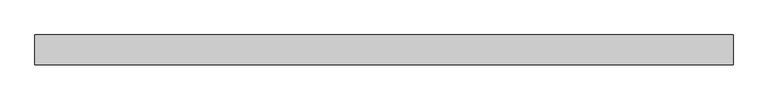
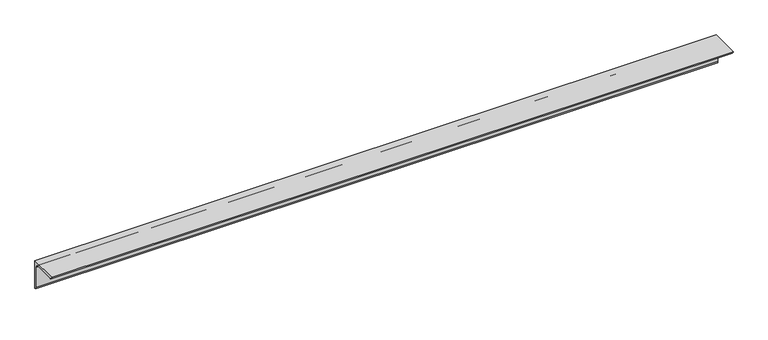
"""IFC4 building model written with IfcOpenShell, lengths in millimetres: beam geometry, 0912_Steel Framing_L-KSD3502 : H_SB_AR_S04_L-130x130x12_KBR1."""

import ifcopenshell
import ifcopenshell.guid

model = None  # the IFC model being written
_history = None  # IfcOwnerHistory: only IFC2X3 demands one
_inside = {}  # id of a spatial element -> (the spatial element, [elements in it])
_under = {}  # id of a project, library or spatial element -> (it, [spatial elements below it])
_declared = {}  # id of a project -> (the project, [libraries it declares])
_typed = {}  # id of a type object -> (the type object, [elements of that type])
_made_of = {}  # id of a material, layer set ... -> (it, [elements and type objects made of it])


def new_model(schema):
    """Start an empty IFC model of exactly this schema.

    Asked for "IFC4X3", IfcOpenShell would pick the latest addendum, in which some entities
    have other attributes; the version numbers below select the first issue.
    IFC2X3 requires an IfcOwnerHistory on every rooted entity: one is made here for all.
    """
    global model, _history
    if schema == "IFC4X3":
        model = ifcopenshell.file(schema_version=(4, 3, 0, 0))
    else:
        model = ifcopenshell.file(schema=schema)
    _inside.clear()
    _under.clear()
    _declared.clear()
    _typed.clear()
    _made_of.clear()
    _history = None
    if model.schema == "IFC2X3":
        org = make("IfcOrganization", Name="unknown")
        user = make(
            "IfcPersonAndOrganization",
            ThePerson=make("IfcPerson", FamilyName="unknown"),
            TheOrganization=org,
        )
        app = make(
            "IfcApplication",
            ApplicationDeveloper=org,
            Version="unknown",
            ApplicationFullName="unknown",
            ApplicationIdentifier="unknown",
        )
        _history = make(
            "IfcOwnerHistory",
            OwningUser=user,
            OwningApplication=app,
            ChangeAction="ADDED",
            CreationDate=0,
        )
    return model


def make(cls, **values):
    """One entity of the class cls with the attributes given. An attribute that is None is left unset."""
    return model.create_entity(
        cls, **{name: value for name, value in values.items() if value is not None}
    )


def rooted(cls, **values):
    """An entity with a GlobalId (a new one), such as an element, a storey or a relation."""
    return make(cls, GlobalId=ifcopenshell.guid.new(), OwnerHistory=_history, **values)


def si_unit(unit_type, name, prefix=None):
    """IfcSIUnit, for example si_unit("LENGTHUNIT", "METRE", prefix="MILLI")."""
    return make("IfcSIUnit", UnitType=unit_type, Prefix=prefix, Name=name)


def assignment(units):
    """IfcUnitAssignment: the units of a project."""
    return None if units is None else make("IfcUnitAssignment", Units=units)


def point(xyz):
    """IfcCartesianPoint."""
    return None if xyz is None else make("IfcCartesianPoint", Coordinates=xyz)


def direction(xyz):
    """IfcDirection."""
    return None if xyz is None else make("IfcDirection", DirectionRatios=xyz)


def frame(location, z_axis=None, x_axis=None):
    """IfcAxis2Placement3D, a coordinate frame: its origin and axes. An axis left out is left unset."""
    return make(
        "IfcAxis2Placement3D",
        Location=point(location),
        Axis=direction(z_axis),
        RefDirection=direction(x_axis),
    )


def frame_2d(location, x_axis=None):
    """IfcAxis2Placement2D, a coordinate frame in the plane: its origin and x axis."""
    return make(
        "IfcAxis2Placement2D", Location=point(location), RefDirection=direction(x_axis)
    )


def origin():
    """The frame at (0, 0, 0) with its axes left unset."""
    return frame((0.0, 0.0, 0.0))


def place(relative_to, where):
    """IfcLocalPlacement: puts the frame where relative to a parent placement (None: the world)."""
    return make(
        "IfcLocalPlacement", PlacementRelTo=relative_to, RelativePlacement=where
    )


def context(
    kind, dimensions, precision=None, world=None, true_north=None, identifier=None
):
    """IfcGeometricRepresentationContext, for example the 3D "Model" context."""
    return make(
        "IfcGeometricRepresentationContext",
        ContextIdentifier=identifier,
        ContextType=kind,
        CoordinateSpaceDimension=dimensions,
        Precision=precision,
        WorldCoordinateSystem=world,
        TrueNorth=true_north,
    )


def project(units=None, contexts=None):
    """IfcProject with its units and contexts."""
    return rooted(
        "IfcProject",
        Name="project",
        RepresentationContexts=contexts,
        UnitsInContext=assignment(units),
    )


def spatial(cls, under=None, at=None, **own):
    """A site, building, storey or space (cls), placed at a placement, below another one or the project."""
    s = rooted(cls, ObjectPlacement=at, **own)
    if under is not None:
        _under.setdefault(under.id(), (under, []))[1].append(s)
    return s


def polyline(points):
    """IfcPolyline through the points."""
    return make("IfcPolyline", Points=[point(p) for p in points])


def circle_curve(where, radius):
    """IfcCircle in the frame where."""
    return make("IfcCircle", Position=where, Radius=radius)


def trimmed(basis, trim1, trim2, sense, master):
    """IfcTrimmedCurve: the piece of a basis curve between two trims."""
    return make(
        "IfcTrimmedCurve",
        BasisCurve=basis,
        Trim1=trim1,
        Trim2=trim2,
        SenseAgreement=sense,
        MasterRepresentation=master,
    )


def segment(curve, same_sense, transition):
    """IfcCompositeCurveSegment."""
    return make(
        "IfcCompositeCurveSegment",
        Transition=transition,
        SameSense=same_sense,
        ParentCurve=curve,
    )


def composite_curve(segments, self_intersect=None):
    """IfcCompositeCurve: segments joined end to end."""
    return make("IfcCompositeCurve", Segments=segments, SelfIntersect=self_intersect)


def outline(outer, holes=None, kind="AREA"):
    """IfcArbitraryClosedProfileDef: a profile drawn as a closed curve; with holes, ...WithVoids."""
    if holes is None:
        return make("IfcArbitraryClosedProfileDef", ProfileType=kind, OuterCurve=outer)
    return make(
        "IfcArbitraryProfileDefWithVoids",
        ProfileType=kind,
        OuterCurve=outer,
        InnerCurves=holes,
    )


def extrude(swept, where, along, depth):
    """IfcExtrudedAreaSolid: the profile swept, set in the frame where, extruded along a direction by depth."""
    return make(
        "IfcExtrudedAreaSolid",
        SweptArea=swept,
        Position=where,
        ExtrudedDirection=direction(along),
        Depth=depth,
    )


def shape(context_of_items, identifier, shape_type, items):
    """IfcShapeRepresentation: the items that make up one representation, for example the "Body"."""
    return make(
        "IfcShapeRepresentation",
        ContextOfItems=context_of_items,
        RepresentationIdentifier=identifier,
        RepresentationType=shape_type,
        Items=items,
    )


def source(mapping_origin, context_of_items, identifier, shape_type, items):
    """IfcRepresentationMap: a shape defined once, which mapped items show again and again."""
    return make(
        "IfcRepresentationMap",
        MappingOrigin=mapping_origin,
        MappedRepresentation=shape(context_of_items, identifier, shape_type, items),
    )


def transform(
    local_origin,
    x_axis=None,
    y_axis=None,
    z_axis=None,
    scale=None,
    scale2=None,
    scale3=None,
    uniform=True,
):
    """IfcCartesianTransformationOperator3D, or its non-uniform kind. x_axis, y_axis, z_axis: its Axis1, 2, 3."""
    if uniform:
        return make(
            "IfcCartesianTransformationOperator3D",
            Axis1=direction(x_axis),
            Axis2=direction(y_axis),
            LocalOrigin=point(local_origin),
            Scale=scale,
            Axis3=direction(z_axis),
        )
    return make(
        "IfcCartesianTransformationOperator3DnonUniform",
        Axis1=direction(x_axis),
        Axis2=direction(y_axis),
        LocalOrigin=point(local_origin),
        Scale=scale,
        Axis3=direction(z_axis),
        Scale2=scale2,
        Scale3=scale3,
    )


def mapped(mapping_source, mapping_target):
    """IfcMappedItem: shows the shape of a source again, moved by a transform."""
    return make(
        "IfcMappedItem", MappingSource=mapping_source, MappingTarget=mapping_target
    )


def made_of(thing, what):
    """Note that an element or type object is made of a material, layer set ...; save() writes the relation."""
    if what is not None:
        _made_of.setdefault(what.id(), (what, []))[1].append(thing)
    return thing


def element(
    cls,
    number,
    at=None,
    inside=None,
    cuts=None,
    type_object=None,
    material=None,
    context=None,
    identifier="Body",
    shape_type=None,
    held_by="IfcProductDefinitionShape",
    body=None,
    shapes=None,
    **own,
):
    """One element of the class cls, such as IfcWall. Its Tag is "e" and its number.

    at: its placement. inside: the storey or other place that contains it. cuts: it is an
    opening in that element (IfcRelVoidsElement). A single representation is given by context,
    identifier, shape_type and body (its items); several are given by shapes. held_by: the class
    of the entity that holds the representations. save() writes the other relations.
    """
    e = rooted(cls, Tag="e%d" % number, ObjectPlacement=at, **own)
    if body is not None:
        shapes = [shape(context, identifier, shape_type, body)]
    if shapes is not None:
        e.Representation = make(held_by, Representations=shapes)
    if inside is not None:
        _inside.setdefault(inside.id(), (inside, []))[1].append(e)
    if cuts is not None:
        rooted(
            "IfcRelVoidsElement", RelatingBuildingElement=cuts, RelatedOpeningElement=e
        )
    if type_object is not None:
        _typed.setdefault(type_object.id(), (type_object, []))[1].append(e)
    return made_of(e, material)


def aggregate(whole, parts):
    """IfcRelAggregates: a whole, such as a stair, and the parts it consists of."""
    return rooted("IfcRelAggregates", RelatingObject=whole, RelatedObjects=parts)


def save(model, path):
    """Write the relations noted so far, then the file.

    IfcRelAggregates (storeys below a building ...), IfcRelContainedInSpatialStructure (elements
    in a storey), IfcRelDefinesByType, IfcRelAssociatesMaterial and IfcRelDeclares: one each for
    every whole, place, type object, material and project.
    """
    for whole, parts in _under.values():
        aggregate(whole, parts)
    for where, things in _inside.values():
        rooted(
            "IfcRelContainedInSpatialStructure",
            RelatedElements=things,
            RelatingStructure=where,
        )
    for kind, things in _typed.values():
        rooted("IfcRelDefinesByType", RelatedObjects=things, RelatingType=kind)
    for what, things in _made_of.values():
        rooted("IfcRelAssociatesMaterial", RelatedObjects=things, RelatingMaterial=what)
    for by, libraries in _declared.values():
        rooted("IfcRelDeclares", RelatingContext=by, RelatedDefinitions=libraries)
    model.write(path)


def beam_d8285e93(model_context):
    return source(origin(), model_context, "Body", "SweptSolid", [
        extrude(outline(composite_curve([segment(polyline([(36.4, 36.4), (36.4, -93.6)]), True, "CONTINUOUS"), segment(trimmed(circle_curve(frame_2d((36.4, -81.6)), 12.0), [point((36.4, -93.6))], [point((24.4, -81.6))], False, "CARTESIAN"), True, "CONTINUOUS"), segment(polyline([(24.4, -81.6), (24.4, 12.4)]), True, "CONTINUOUS"), segment(trimmed(circle_curve(frame_2d((12.4, 12.4)), 12.0), [point((24.4, 12.4))], [point((12.4, 24.4))], True, "CARTESIAN"), True, "CONTINUOUS"), segment(polyline([(12.4, 24.4), (-81.6, 24.4)]), True, "CONTINUOUS"), segment(trimmed(circle_curve(frame_2d((-81.6, 36.4)), 12.0), [point((-81.6, 24.4))], [point((-93.6, 36.4))], False, "CARTESIAN"), True, "CONTINUOUS"), segment(polyline([(-93.6, 36.4), (36.4, 36.4)]), True, "CONTINUOUS")], self_intersect=False)), frame((-1519.4237854, 0.0, 0.0), z_axis=(1.0, 0.0, 0.0), x_axis=(0.0, 1.0, 0.0)), (0.0, 0.0, 1.0), 3039.6020843),
    ])


if __name__ == "__main__":
    model = new_model("IFC4")
    model_context = context("Model", 3, world=origin())
    ifc_project = project(units=[si_unit("LENGTHUNIT", "METRE", prefix="MILLI")], contexts=[model_context])
    site = spatial("IfcSite", under=ifc_project)
    building = spatial("IfcBuilding", under=site)
    placement = place(None, origin())
    beam_shape = beam_d8285e93(model_context)
    element("IfcBeam", 1, ObjectType="0912_Steel Framing_L-KSD3502 : H_SB_AR_S04_L-130x130x12_KBR1", at=placement, inside=building, context=model_context, shape_type="MappedRepresentation", body=[
        mapped(beam_shape, transform((0.0, 0.0, 0.0), x_axis=(1.0, 0.0, 0.0), y_axis=(0.0, 1.0, 0.0), z_axis=(0.0, 0.0, 1.0))),
    ])
    save(model, "model.ifc")

# Revit data of these elements
# Type "0912_Steel Framing_L-KSD3502 : H_SB_AR_S04_L-130x130x12_KBR1"
#   k = 25 mm
#   Perimeter = 0.52 m²/m
#   Nominal Weight = 23.40 kgf/m
#   Length [instance default] = 1000 mm
#   b = 130 mm
#   d = 130 mm
#   t = 12 mm
#   x = 36.4 mm
#   y = 36.4 mm
#   A = 2976.00 m²
#   Structural Material [instance default] = Steel, 45-345
# Element 1 (IfcBeam, "0912_Steel Framing_L-KSD3502 : H_SB_AR_S04_L-130x130x12_KBR1")
#   Materials on its faces: "Steel, 45-345"
# Materials
#   "Steel, 45-345": class "Metal", colour RGB 189 187 185, transparency 0, Description = "Steel 345 MPa", Cost = 0
